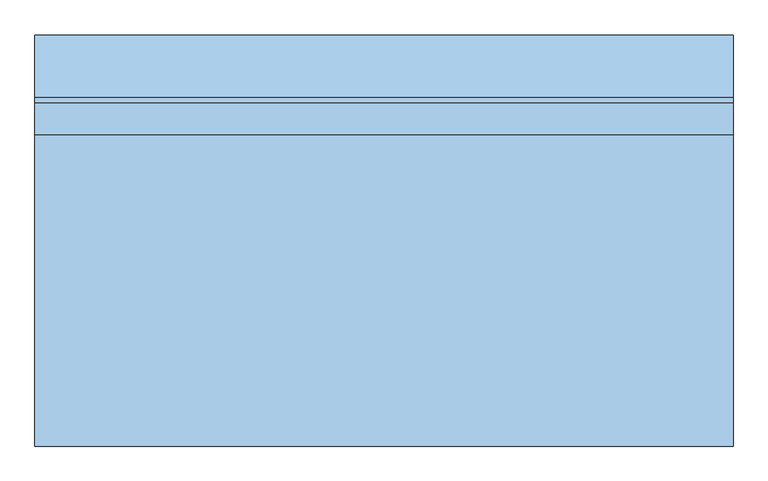
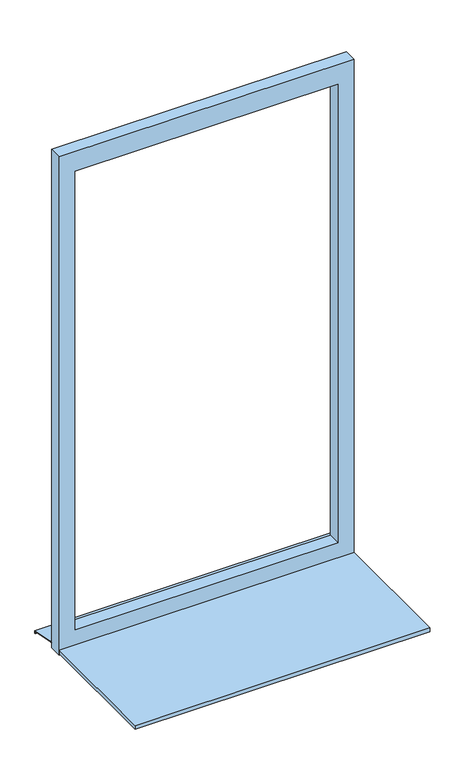
"""IFC4 building model written with IfcOpenShell, lengths in millimetres: window geometry, Fenster - Festverglasung : Feste Verglasung 1.25x2."""

from ifc_helpers import new_model, si_unit, frame, origin, place, context, project, spatial, polyline, outline, extrude, source, transform, mapped, element, save


def window_5bcb729f(model_context):
    return source(origin(), model_context, "Body", "SweptSolid", [
        extrude(outline(polyline([(3000.0, 560.0), (3000.0, -560.0), (1000.0, -560.0), (1000.0, 560.0), (3000.0, 560.0)]), holes=[polyline([(2920.0, 500.0), (1080.0, 500.0), (1080.0, -500.0), (2920.0, -500.0), (2920.0, 500.0)])]), frame((0.0, 170.0, 0.0), z_axis=(0.0, 1.0, 0.0), x_axis=(0.0, 0.0, 1.0)), (0.0, 0.0, 1.0), 50.0),
        extrude(outline(polyline([(-560.0, -330.0), (-560.0, 170.0), (560.0, 170.0), (560.0, -330.0), (-560.0, -330.0)])), frame((0.0, 0.0, 1005.0), z_axis=(0.0, 0.0, 1.0), x_axis=(1.0, 0.0, 0.0)), (0.0, 0.0, 1.0), 15.0),
        extrude(outline(polyline([(230.0221543, 1020.0), (330.0, 1000.0), (330.0, 990.0), (328.0, 990.0), (328.0, 998.3604634), (229.8240723, 1018.0), (220.0, 1018.0), (220.0, 1020.0), (230.0221543, 1020.0)])), frame((-560.0, 0.0, 0.0), z_axis=(1.0, 0.0, 0.0), x_axis=(0.0, 1.0, 0.0)), (0.0, 0.0, 1.0), 1120.0),
    ])


if __name__ == "__main__":
    model = new_model("IFC4")
    model_context = context("Model", 3, world=origin())
    ifc_project = project(units=[si_unit("LENGTHUNIT", "METRE", prefix="MILLI")], contexts=[model_context])
    site = spatial("IfcSite", under=ifc_project)
    building = spatial("IfcBuilding", under=site)
    placement = place(None, origin())
    window_shape = window_5bcb729f(model_context)
    element("IfcWindow", 1, ObjectType="Fenster - Festverglasung : Feste Verglasung 1.25x2", at=placement, inside=building, context=model_context, shape_type="MappedRepresentation", body=[
        mapped(window_shape, transform((0.0, 0.0, 0.0), x_axis=(1.0, 0.0, 0.0), y_axis=(0.0, 1.0, 0.0), z_axis=(0.0, 0.0, 1.0))),
    ])
    save(model, "model.ifc")

# Revit data of these elements
# Type "Fenster - Festverglasung : Feste Verglasung 1.25x2"
#   Type Mark = "54"
#   Operation = "SinglePanel"
#   Keynote = "16.05.01"
#   Visual Light Transmittance = 0.9
#   Solar Heat Gain Coefficient = 0.78
#   Rough Width = 1.120 m
#   Rough Height = 2.000 m
#   Heat Transfer Coefficient (U) = 3.6886 W/(m²·K)
#   Rahmentiefe = 0.050 m
#   Rahmenhöhe unten = 0.080 m
#   Höhe oberer  Rahmen = 0.080 m
#   Rahmenbreite = 0.060 m
#   Height = 2.000 m
#   Einbautiefe (von außen) [instance default] = 0.080 m
#   Width = 1.120 m
#   Wall Closure = 2
#   Bild [instance default] = none
#   Glas [instance default] = none
#   Innere Fensterbank [instance default] = none
#   Äußere Fensterbank [instance default] = none
#   Construction Type Id = ""
#   Analytic Construction = (empty or 0)
# Element 1 (IfcWindow, "Fenster - Festverglasung : Feste Verglasung 1.25x2")
#   Materials on its faces: "Kunststoff - Weiß", "Holz - Birke"
# Materials
#   "Kunststoff - Weiß": class "Kunststoff", colour RGB 249 249 249, transparency 0, Cost = 0
#   "Holz - Birke": class "Holz", colour RGB 213 164 103, transparency 0, Cost = 0
